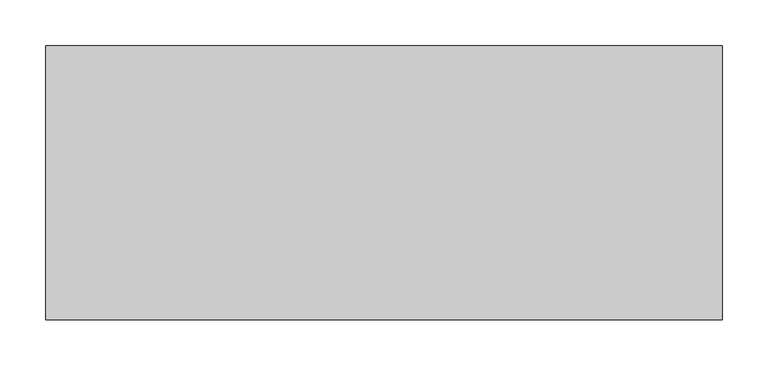
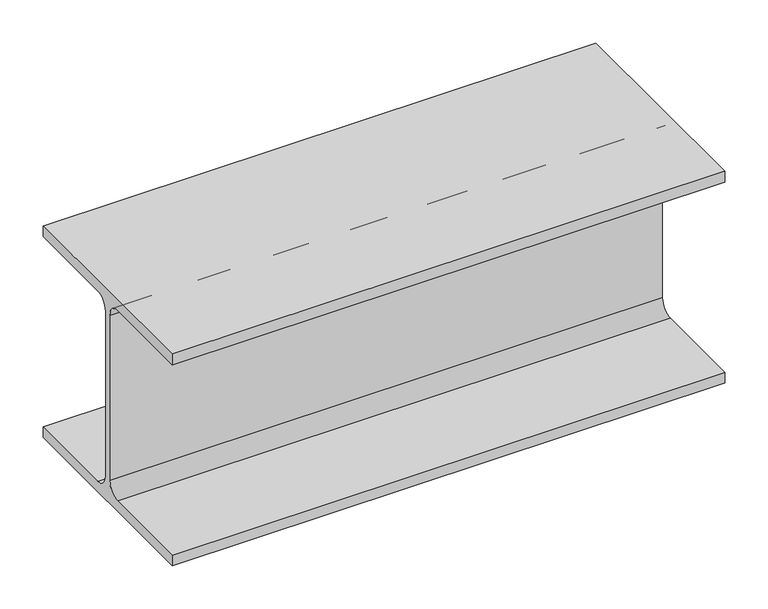
"""IFC4 building model written with IfcOpenShell, lengths in millimetres: beam geometry, 0912_Steel Framing_H-KSD3502 : H_SB_ASB_H-300x300x10x15."""

from ifc_helpers import new_model, si_unit, point, frame, frame_2d, origin, place, context, project, spatial, polyline, circle_curve, trimmed, segment, composite_curve, outline, extrude, source, transform, mapped, element, save


def beam_a46f469d(model_context):
    return source(origin(), model_context, "Body", "SweptSolid", [
        extrude(outline(composite_curve([segment(polyline([(150.0, -135.0), (150.0, -150.0), (-150.0, -150.0), (-150.0, -135.0), (-23.0, -135.0)]), True, "CONTINUOUS"), segment(trimmed(circle_curve(frame_2d((-23.0, -117.0)), 18.0), [point((-23.0, -135.0))], [point((-5.0, -117.0))], True, "CARTESIAN"), True, "CONTINUOUS"), segment(polyline([(-5.0, -117.0), (-5.0, 117.0)]), True, "CONTINUOUS"), segment(trimmed(circle_curve(frame_2d((-23.0, 117.0)), 18.0), [point((-5.0, 117.0))], [point((-23.0, 135.0))], True, "CARTESIAN"), True, "CONTINUOUS"), segment(polyline([(-23.0, 135.0), (-150.0, 135.0), (-150.0, 150.0), (150.0, 150.0), (150.0, 135.0), (23.0, 135.0)]), True, "CONTINUOUS"), segment(trimmed(circle_curve(frame_2d((23.0, 117.0)), 18.0), [point((23.0, 135.0))], [point((5.0, 117.0))], True, "CARTESIAN"), True, "CONTINUOUS"), segment(polyline([(5.0, 117.0), (5.0, -117.0)]), True, "CONTINUOUS"), segment(trimmed(circle_curve(frame_2d((23.0, -117.0)), 18.0), [point((5.0, -117.0))], [point((23.0, -135.0))], True, "CARTESIAN"), True, "CONTINUOUS"), segment(polyline([(23.0, -135.0), (150.0, -135.0)]), True, "CONTINUOUS")], self_intersect=False)), frame((-502.4937811, 0.0, 0.0), z_axis=(1.0, 0.0, 0.0), x_axis=(0.0, 1.0, 0.0)), (0.0, 0.0, 1.0), 740.4687108),
    ])


if __name__ == "__main__":
    model = new_model("IFC4")
    model_context = context("Model", 3, world=origin())
    ifc_project = project(units=[si_unit("LENGTHUNIT", "METRE", prefix="MILLI")], contexts=[model_context])
    site = spatial("IfcSite", under=ifc_project)
    building = spatial("IfcBuilding", under=site)
    placement = place(None, origin())
    beam_shape = beam_a46f469d(model_context)
    element("IfcBeam", 1, ObjectType="0912_Steel Framing_H-KSD3502 : H_SB_ASB_H-300x300x10x15", at=placement, inside=building, context=model_context, shape_type="MappedRepresentation", body=[
        mapped(beam_shape, transform((0.0, 0.0, 0.0), x_axis=(1.0, 0.0, 0.0), y_axis=(0.0, 1.0, 0.0), z_axis=(0.0, 0.0, 1.0))),
    ])
    save(model, "model.ifc")

# Revit data of these elements
# Type "0912_Steel Framing_H-KSD3502 : H_SB_ASB_H-300x300x10x15"
#   H_WM Code_1 = "S01AA001-00001 | Main Steel Structure Fabrication Work | Shelter/Building | Heavy Steel - Standard (Weight≥90KG/M) | Material: (   )"
#   H_WM Code_2 = "S03AA027-00001 | Main Steel Structure Erection Work | Shelter/Building | Heavy Steel (Weight≥90KG/M) | Material: (   )"
#   H_WM Code_3 = "S01AA010-00001 | Main Steel Structure Fabrication Work | Shelter/Building | Steel Painting/Coating | for Non-Fireproofed Steel Surface, Surface Preparation, Primer, Second & Final Coat | Material: (   )"
#   H_Q'ty Cal Type Tag = "SB-Q2"
#   Width = 30.0 cm
#   Web Thickness = 1.0 cm
#   Web Fillet = 1.8 cm
#   Warping Constant = 1370000.0 cm⁶
#   W = 0
#   Torsional Moment of Inertia = 77.00 cm⁴
#   Section Area = 119.8 cm²
#   Plastic Modulus weak axis = 684.0 cm³
#   Plastic Modulus strong axis = 1500.0 cm³
#   Perimeter = 1.75 m²/m
#   Nominal Weight = 94.00 kgf/m
#   Moment of Inertia weak axis = 6750.00 cm⁴
#   Moment of Inertia strong axis = 20400.00 cm⁴
#   Height = 30.0 cm
#   Flange Thickness = 1.5 cm
#   Elastic Modulus weak axis = 450.0 cm³
#   Elastic Modulus strong axis = 1360.0 cm³
#   Centroid Vertical = 15.0 cm
#   Centroid Horizontal = 15.0 cm
#   Ix = 204000000
#   Length [instance default] = 1.5240 m
#   Zx = 1500000
#   b = 0.3000 m
#   h = 0.3000 m
#   r = 0.0180 m
#   s = 0.0100 m
#   t = 0.0150 m
#   A = 0.01198 m²
#   Structural Material [instance default] = Steel, 45-345
#   Assembly Code = ""
# Element 1 (IfcBeam, "0912_Steel Framing_H-KSD3502 : H_SB_ASB_H-300x300x10x15")
#   Structural Material = none
# Materials
#   "Steel, 45-345": class "Metal", colour RGB 189 187 185, transparency 0, Description = "Steel 345 MPa", Cost = 0
